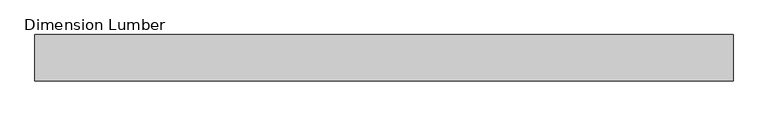
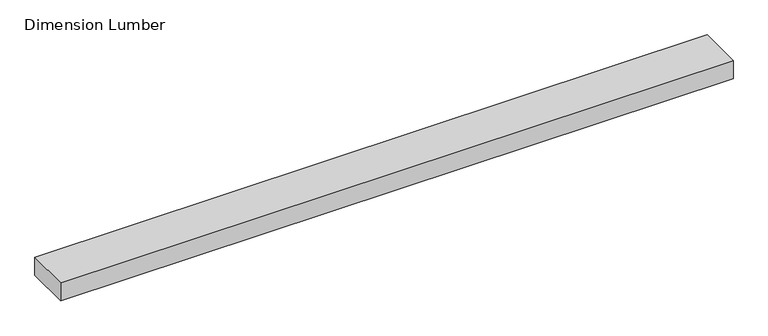
"""IFC4 building model written with IfcOpenShell, lengths in millimetres: beam geometry, Dimension Lumber : Top Supporting Lumbers."""

from ifc_helpers import new_model, si_unit, frame, origin, place, context, project, spatial, polyline, outline, extrude, source, transform, mapped, element, save


def dimension_lumber_e4f6bc88(model_context):
    return source(origin(), model_context, "Body", "SweptSolid", [
        extrude(outline(polyline([(5029.99375, 44.45), (5029.99375, -44.45), (3696.49375, -44.45), (3696.49375, 44.45), (5029.99375, 44.45)])), frame((0.0, 0.0, -19.05), z_axis=(0.0, 0.0, 1.0), x_axis=(1.0, 0.0, 0.0)), (0.0, 0.0, 1.0), 38.1),
    ])


if __name__ == "__main__":
    model = new_model("IFC4")
    model_context = context("Model", 3, world=origin())
    ifc_project = project(units=[si_unit("LENGTHUNIT", "METRE", prefix="MILLI")], contexts=[model_context])
    site = spatial("IfcSite", under=ifc_project)
    building = spatial("IfcBuilding", under=site)
    placement = place(None, origin())
    dimension_lumber_shape = dimension_lumber_e4f6bc88(model_context)
    element("IfcBeam", 1, ObjectType="Dimension Lumber : Top Supporting Lumbers", at=placement, inside=building, context=model_context, shape_type="MappedRepresentation", body=[
        mapped(dimension_lumber_shape, transform((0.0, 0.0, 0.0), x_axis=(1.0, 0.0, 0.0), y_axis=(0.0, 1.0, 0.0), z_axis=(0.0, 0.0, 1.0))),
    ])
    save(model, "model.ifc")

# Revit data of these elements
# Type "Dimension Lumber : Top Supporting Lumbers"
#   Assembly Code = "B10"
#   A = 0.0364583 SF
#   Length [instance default] = 5' - 0"
#   b = 0' - 3 1/2"
#   d = 0' - 1 1/2"
#   Structural Material [instance default] = Softwood, Lumber
# Element 1 (IfcBeam, "Dimension Lumber : Top Supporting Lumbers")
#   Structural Material = Douglas Fir #2
#   Materials on its faces: "Douglas Fir #2"
# Materials
#   "Softwood, Lumber": class "Wood", colour RGB 223 192 134, transparency 0, Description = "Pinus Echinata", Cost = 0
#   "Douglas Fir #2": class "Wood", colour RGB 223 192 134, transparency 0, Description = "Pinus Echinata", Cost = 0
